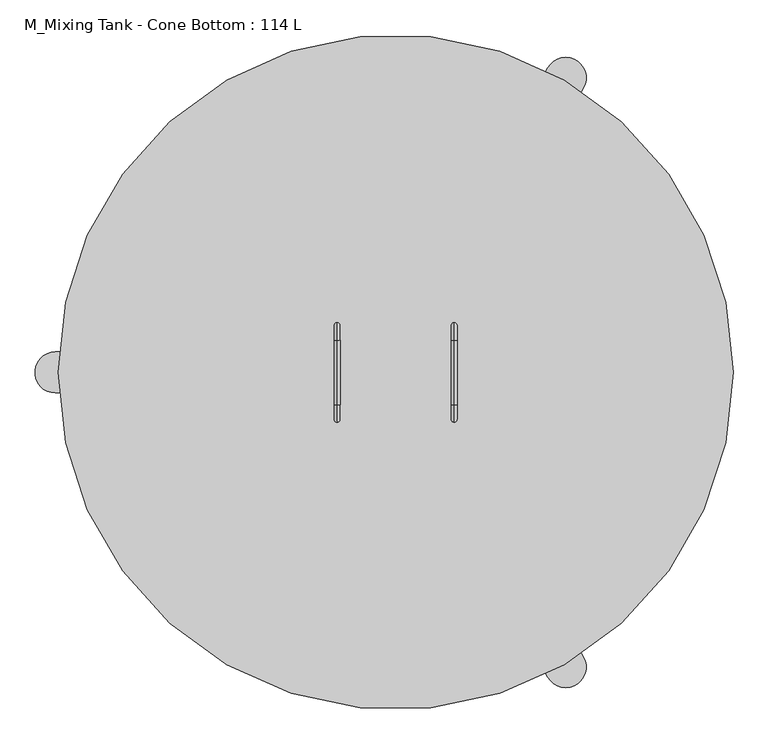
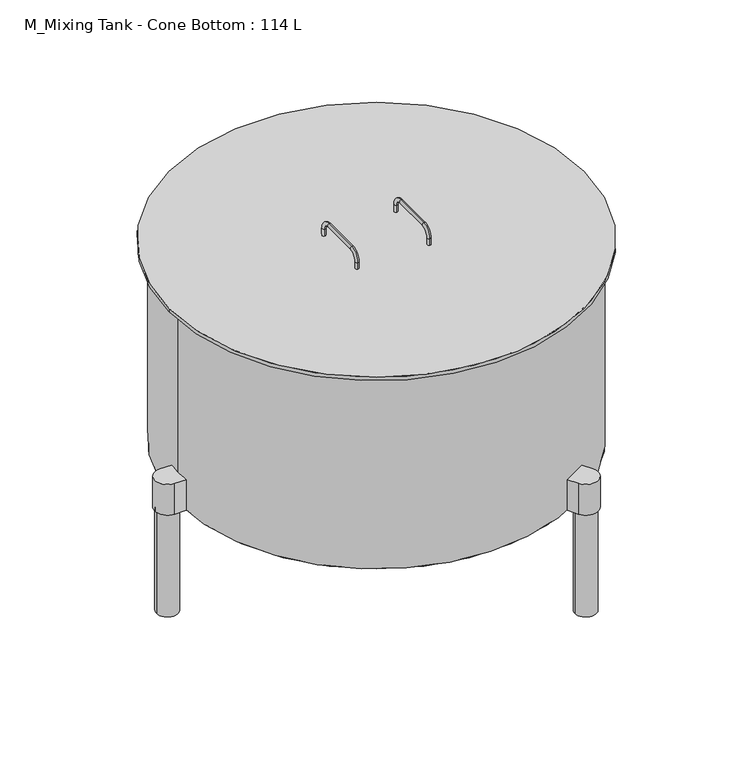
"""IFC4 building model written with IfcOpenShell, lengths in millimetres: proxy geometry, M_Mixing Tank - Cone Bottom : 114 L."""

import ifcopenshell
import ifcopenshell.guid

model = None  # the IFC model being written
_history = None  # IfcOwnerHistory: only IFC2X3 demands one
_inside = {}  # id of a spatial element -> (the spatial element, [elements in it])
_under = {}  # id of a project, library or spatial element -> (it, [spatial elements below it])
_declared = {}  # id of a project -> (the project, [libraries it declares])
_typed = {}  # id of a type object -> (the type object, [elements of that type])
_made_of = {}  # id of a material, layer set ... -> (it, [elements and type objects made of it])


def new_model(schema):
    """Start an empty IFC model of exactly this schema.

    Asked for "IFC4X3", IfcOpenShell would pick the latest addendum, in which some entities
    have other attributes; the version numbers below select the first issue.
    IFC2X3 requires an IfcOwnerHistory on every rooted entity: one is made here for all.
    """
    global model, _history
    if schema == "IFC4X3":
        model = ifcopenshell.file(schema_version=(4, 3, 0, 0))
    else:
        model = ifcopenshell.file(schema=schema)
    _inside.clear()
    _under.clear()
    _declared.clear()
    _typed.clear()
    _made_of.clear()
    _history = None
    if model.schema == "IFC2X3":
        org = make("IfcOrganization", Name="unknown")
        user = make(
            "IfcPersonAndOrganization",
            ThePerson=make("IfcPerson", FamilyName="unknown"),
            TheOrganization=org,
        )
        app = make(
            "IfcApplication",
            ApplicationDeveloper=org,
            Version="unknown",
            ApplicationFullName="unknown",
            ApplicationIdentifier="unknown",
        )
        _history = make(
            "IfcOwnerHistory",
            OwningUser=user,
            OwningApplication=app,
            ChangeAction="ADDED",
            CreationDate=0,
        )
    return model


def make(cls, **values):
    """One entity of the class cls with the attributes given. An attribute that is None is left unset."""
    return model.create_entity(
        cls, **{name: value for name, value in values.items() if value is not None}
    )


def rooted(cls, **values):
    """An entity with a GlobalId (a new one), such as an element, a storey or a relation."""
    return make(cls, GlobalId=ifcopenshell.guid.new(), OwnerHistory=_history, **values)


def si_unit(unit_type, name, prefix=None):
    """IfcSIUnit, for example si_unit("LENGTHUNIT", "METRE", prefix="MILLI")."""
    return make("IfcSIUnit", UnitType=unit_type, Prefix=prefix, Name=name)


def assignment(units):
    """IfcUnitAssignment: the units of a project."""
    return None if units is None else make("IfcUnitAssignment", Units=units)


def point(xyz):
    """IfcCartesianPoint."""
    return None if xyz is None else make("IfcCartesianPoint", Coordinates=xyz)


def direction(xyz):
    """IfcDirection."""
    return None if xyz is None else make("IfcDirection", DirectionRatios=xyz)


def frame(location, z_axis=None, x_axis=None):
    """IfcAxis2Placement3D, a coordinate frame: its origin and axes. An axis left out is left unset."""
    return make(
        "IfcAxis2Placement3D",
        Location=point(location),
        Axis=direction(z_axis),
        RefDirection=direction(x_axis),
    )


def frame_2d(location, x_axis=None):
    """IfcAxis2Placement2D, a coordinate frame in the plane: its origin and x axis."""
    return make(
        "IfcAxis2Placement2D", Location=point(location), RefDirection=direction(x_axis)
    )


def origin():
    """The frame at (0, 0, 0) with its axes left unset."""
    return frame((0.0, 0.0, 0.0))


def origin_with_axes():
    """The frame at (0, 0, 0) with the z axis (0, 0, 1) and the x axis (1, 0, 0) written out."""
    return frame((0.0, 0.0, 0.0), z_axis=(0.0, 0.0, 1.0), x_axis=(1.0, 0.0, 0.0))


def origin_2d():
    """The frame at (0, 0) in the plane with its x axis left unset."""
    return frame_2d((0.0, 0.0))


def place(relative_to, where):
    """IfcLocalPlacement: puts the frame where relative to a parent placement (None: the world)."""
    return make(
        "IfcLocalPlacement", PlacementRelTo=relative_to, RelativePlacement=where
    )


def context(
    kind, dimensions, precision=None, world=None, true_north=None, identifier=None
):
    """IfcGeometricRepresentationContext, for example the 3D "Model" context."""
    return make(
        "IfcGeometricRepresentationContext",
        ContextIdentifier=identifier,
        ContextType=kind,
        CoordinateSpaceDimension=dimensions,
        Precision=precision,
        WorldCoordinateSystem=world,
        TrueNorth=true_north,
    )


def project(units=None, contexts=None):
    """IfcProject with its units and contexts."""
    return rooted(
        "IfcProject",
        Name="project",
        RepresentationContexts=contexts,
        UnitsInContext=assignment(units),
    )


def spatial(cls, under=None, at=None, **own):
    """A site, building, storey or space (cls), placed at a placement, below another one or the project."""
    s = rooted(cls, ObjectPlacement=at, **own)
    if under is not None:
        _under.setdefault(under.id(), (under, []))[1].append(s)
    return s


def polyline(points):
    """IfcPolyline through the points."""
    return make("IfcPolyline", Points=[point(p) for p in points])


def circle_curve(where, radius):
    """IfcCircle in the frame where."""
    return make("IfcCircle", Position=where, Radius=radius)


def ellipse_curve(where, semi_axis1, semi_axis2):
    """IfcEllipse in the frame where."""
    return make(
        "IfcEllipse", Position=where, SemiAxis1=semi_axis1, SemiAxis2=semi_axis2
    )


def trimmed(basis, trim1, trim2, sense, master):
    """IfcTrimmedCurve: the piece of a basis curve between two trims."""
    return make(
        "IfcTrimmedCurve",
        BasisCurve=basis,
        Trim1=trim1,
        Trim2=trim2,
        SenseAgreement=sense,
        MasterRepresentation=master,
    )


def segment(curve, same_sense, transition):
    """IfcCompositeCurveSegment."""
    return make(
        "IfcCompositeCurveSegment",
        Transition=transition,
        SameSense=same_sense,
        ParentCurve=curve,
    )


def composite_curve(segments, self_intersect=None):
    """IfcCompositeCurve: segments joined end to end."""
    return make("IfcCompositeCurve", Segments=segments, SelfIntersect=self_intersect)


def outline(outer, holes=None, kind="AREA"):
    """IfcArbitraryClosedProfileDef: a profile drawn as a closed curve; with holes, ...WithVoids."""
    if holes is None:
        return make("IfcArbitraryClosedProfileDef", ProfileType=kind, OuterCurve=outer)
    return make(
        "IfcArbitraryProfileDefWithVoids",
        ProfileType=kind,
        OuterCurve=outer,
        InnerCurves=holes,
    )


def extrude(swept, where, along, depth):
    """IfcExtrudedAreaSolid: the profile swept, set in the frame where, extruded along a direction by depth."""
    return make(
        "IfcExtrudedAreaSolid",
        SweptArea=swept,
        Position=where,
        ExtrudedDirection=direction(along),
        Depth=depth,
    )


def shape(context_of_items, identifier, shape_type, items):
    """IfcShapeRepresentation: the items that make up one representation, for example the "Body"."""
    return make(
        "IfcShapeRepresentation",
        ContextOfItems=context_of_items,
        RepresentationIdentifier=identifier,
        RepresentationType=shape_type,
        Items=items,
    )


def source(mapping_origin, context_of_items, identifier, shape_type, items):
    """IfcRepresentationMap: a shape defined once, which mapped items show again and again."""
    return make(
        "IfcRepresentationMap",
        MappingOrigin=mapping_origin,
        MappedRepresentation=shape(context_of_items, identifier, shape_type, items),
    )


def transform(
    local_origin,
    x_axis=None,
    y_axis=None,
    z_axis=None,
    scale=None,
    scale2=None,
    scale3=None,
    uniform=True,
):
    """IfcCartesianTransformationOperator3D, or its non-uniform kind. x_axis, y_axis, z_axis: its Axis1, 2, 3."""
    if uniform:
        return make(
            "IfcCartesianTransformationOperator3D",
            Axis1=direction(x_axis),
            Axis2=direction(y_axis),
            LocalOrigin=point(local_origin),
            Scale=scale,
            Axis3=direction(z_axis),
        )
    return make(
        "IfcCartesianTransformationOperator3DnonUniform",
        Axis1=direction(x_axis),
        Axis2=direction(y_axis),
        LocalOrigin=point(local_origin),
        Scale=scale,
        Axis3=direction(z_axis),
        Scale2=scale2,
        Scale3=scale3,
    )


def mapped(mapping_source, mapping_target):
    """IfcMappedItem: shows the shape of a source again, moved by a transform."""
    return make(
        "IfcMappedItem", MappingSource=mapping_source, MappingTarget=mapping_target
    )


def made_of(thing, what):
    """Note that an element or type object is made of a material, layer set ...; save() writes the relation."""
    if what is not None:
        _made_of.setdefault(what.id(), (what, []))[1].append(thing)
    return thing


def element(
    cls,
    number,
    at=None,
    inside=None,
    cuts=None,
    type_object=None,
    material=None,
    context=None,
    identifier="Body",
    shape_type=None,
    held_by="IfcProductDefinitionShape",
    body=None,
    shapes=None,
    **own,
):
    """One element of the class cls, such as IfcWall. Its Tag is "e" and its number.

    at: its placement. inside: the storey or other place that contains it. cuts: it is an
    opening in that element (IfcRelVoidsElement). A single representation is given by context,
    identifier, shape_type and body (its items); several are given by shapes. held_by: the class
    of the entity that holds the representations. save() writes the other relations.
    """
    e = rooted(cls, Tag="e%d" % number, ObjectPlacement=at, **own)
    if body is not None:
        shapes = [shape(context, identifier, shape_type, body)]
    if shapes is not None:
        e.Representation = make(held_by, Representations=shapes)
    if inside is not None:
        _inside.setdefault(inside.id(), (inside, []))[1].append(e)
    if cuts is not None:
        rooted(
            "IfcRelVoidsElement", RelatingBuildingElement=cuts, RelatedOpeningElement=e
        )
    if type_object is not None:
        _typed.setdefault(type_object.id(), (type_object, []))[1].append(e)
    return made_of(e, material)


def aggregate(whole, parts):
    """IfcRelAggregates: a whole, such as a stair, and the parts it consists of."""
    return rooted("IfcRelAggregates", RelatingObject=whole, RelatedObjects=parts)


def save(model, path):
    """Write the relations noted so far, then the file.

    IfcRelAggregates (storeys below a building ...), IfcRelContainedInSpatialStructure (elements
    in a storey), IfcRelDefinesByType, IfcRelAssociatesMaterial and IfcRelDeclares: one each for
    every whole, place, type object, material and project.
    """
    for whole, parts in _under.values():
        aggregate(whole, parts)
    for where, things in _inside.values():
        rooted(
            "IfcRelContainedInSpatialStructure",
            RelatedElements=things,
            RelatingStructure=where,
        )
    for kind, things in _typed.values():
        rooted("IfcRelDefinesByType", RelatedObjects=things, RelatingType=kind)
    for what, things in _made_of.values():
        rooted("IfcRelAssociatesMaterial", RelatedObjects=things, RelatingMaterial=what)
    for by, libraries in _declared.values():
        rooted("IfcRelDeclares", RelatingContext=by, RelatedDefinitions=libraries)
    model.write(path)


def plane_surface(at):
    """IfcPlane: the flat surface through the origin of the frame at, square to its z axis."""
    return make("IfcPlane", Position=at)


def cylinder_surface(at, radius):
    """IfcCylindricalSurface: all points at the distance radius from the z axis of the frame at."""
    return make("IfcCylindricalSurface", Position=at, Radius=radius)


def revolved_surface(curve, axis_point, axis_direction):
    """IfcSurfaceOfRevolution: the curve turned about the line through axis_point along axis_direction."""
    return make(
        "IfcSurfaceOfRevolution",
        SweptCurve=make("IfcArbitraryOpenProfileDef", ProfileType="CURVE", Curve=curve),
        AxisPosition=make("IfcAxis1Placement", Location=point(axis_point), Axis=direction(axis_direction)),
    )


def advanced_brep(points, edges, surfaces, faces):
    """IfcAdvancedBrep: a solid bounded by faces that lie on surfaces and meet in shared edges.

    An edge is (start, end): straight between two places in points (the first is 0);
    or (start, end, curve); or (start, end, curve, False) where it runs against its curve.
    A face is (place in surfaces, loops), or (place, loops, False) where it looks against
    its surface's normal. A loop lists edges by number (the first is 1), with a minus sign
    where the edge is run from its end to its start. The first loop is the outer one.
    """
    corners = [point(p) for p in points]
    vertices = [make("IfcVertexPoint", VertexGeometry=c) for c in corners]
    made = []
    for start, end, *more in edges:
        made.append(
            make(
                "IfcEdgeCurve",
                EdgeStart=vertices[start],
                EdgeEnd=vertices[end],
                EdgeGeometry=more[0] if more else make("IfcPolyline", Points=[corners[start], corners[end]]),
                SameSense=more[1] if len(more) > 1 else True,
            )
        )
    hull = []
    for where, loops, *sense in faces:
        bounds = []
        for j, loop in enumerate(loops):
            ring = [make("IfcOrientedEdge", EdgeElement=made[abs(k) - 1], Orientation=k > 0) for k in loop]
            bounds.append(
                make(
                    "IfcFaceOuterBound" if j == 0 else "IfcFaceBound",
                    Bound=make("IfcEdgeLoop", EdgeList=ring),
                    Orientation=True,
                )
            )
        hull.append(make("IfcAdvancedFace", Bounds=bounds, FaceSurface=surfaces[where], SameSense=sense[0] if sense else True))
    return make("IfcAdvancedBrep", Outer=make("IfcClosedShell", CfsFaces=hull))


def m_mixing_tank_cone_bottom_114_l_11de7092(model_context):
    return source(origin(), model_context, "Body", "SolidModel", [
        extrude(outline(composite_curve([segment(trimmed(circle_curve(origin_2d(), 732.0), [point((-732.0, 0.0))], [point((732.0, 0.0))], False, "CARTESIAN"), True, "CONTINUOUS"), segment(trimmed(circle_curve(origin_2d(), 732.0), [point((732.0, 0.0))], [point((-732.0, 0.0))], False, "CARTESIAN"), True, "CONTINUOUS")], self_intersect=False)), frame((0.0, 0.0, 1108.3), z_axis=(0.0, 0.0, 1.0), x_axis=(1.0, 0.0, 0.0)), (0.0, 0.0, 1.0), 12.7),
        advanced_brep(
        [(700.0, 0.0, 384.0), (-700.0, 0.0, 384.0), (25.0, 0.0, 196.4355653), (-25.0, 0.0, 196.4355653)],
        [
            (0, 1, circle_curve(frame((0.0, 0.0, 384.0), z_axis=(0.0, 0.0, 1.0), x_axis=(1.0, 0.0, 0.0)), 700.0)),
            (1, 0, circle_curve(frame((0.0, 0.0, 384.0), z_axis=(0.0, 0.0, 1.0), x_axis=(-1.0, 0.0, 0.0)), 700.0)),
            (2, 3, circle_curve(frame((0.0, 0.0, 196.4355653), z_axis=(0.0, 0.0, -1.0), x_axis=(-1.0, 0.0, 0.0)), 25.0)),
            (3, 2, circle_curve(frame((0.0, 0.0, 196.4355653), z_axis=(0.0, 0.0, -1.0), x_axis=(1.0, 0.0, 0.0)), 25.0)),
            (3, 1),
            (0, 2),
        ],
        [
            plane_surface(frame((0.0, 0.0, 384.0), z_axis=(0.0, 0.0, 1.0), x_axis=(0.0, 1.0, 0.0))),
            plane_surface(frame((0.0, 0.0, 196.4355653), z_axis=(0.0, 0.0, -1.0), x_axis=(0.0, 1.0, 0.0))),
            revolved_surface(polyline([(-24.99999994858913, 0.0, 196.4355653), (-700.0, 0.0, 384.0)]), (0.0, 0.0, 189.4887344), (0.0, 0.0, 1.0)),
            revolved_surface(polyline([(24.99999994858913, 0.0, 196.4355653), (700.0, 0.0, 384.0)]), (0.0, 0.0, 189.4887344), (0.0, 0.0, 1.0)),
        ],
        [
            (0, [[1, 2]]),
            (1, [[3, 4]]),
            (2, [[-4, 5, -1, 6]]),
            (3, [[-3, -6, -2, -5]]),
        ],
    ),
        extrude(outline(composite_curve([segment(trimmed(circle_curve(origin_2d(), 25.0), [point((-25.0, 0.0))], [point((25.0, 0.0))], False, "CARTESIAN"), True, "CONTINUOUS"), segment(trimmed(circle_curve(origin_2d(), 25.0), [point((25.0, 0.0))], [point((-25.0, 0.0))], False, "CARTESIAN"), True, "CONTINUOUS")], self_intersect=False)), frame((0.0, 0.0, 167.0668153), z_axis=(0.0, 0.0, 1.0), x_axis=(1.0, 0.0, 0.0)), (0.0, 0.0, 1.0), 29.36875),
        extrude(outline(composite_curve([segment(trimmed(circle_curve(origin_2d(), 700.0), [point((-700.0, 0.0))], [point((700.0, 0.0))], False, "CARTESIAN"), True, "CONTINUOUS"), segment(trimmed(circle_curve(origin_2d(), 700.0), [point((700.0, 0.0))], [point((-700.0, 0.0))], False, "CARTESIAN"), True, "CONTINUOUS")], self_intersect=False)), frame((0.0, 0.0, 384.0), z_axis=(0.0, 0.0, 1.0), x_axis=(1.0, 0.0, 0.0)), (0.0, 0.0, 1.0), 724.3),
        extrude(outline(composite_curve([segment(polyline([(407.4948292, 616.901748), (387.1653983, 581.6901407)]), True, "CONTINUOUS"), segment(trimmed(circle_curve(origin_2d(), 698.7563706), [point((387.1653983, 581.6901407))], [point((310.1757399, 626.1401407))], True, "CARTESIAN"), True, "CONTINUOUS"), segment(polyline([(310.1757399, 626.1401407), (330.5051708, 661.351748)]), True, "CONTINUOUS"), segment(trimmed(circle_curve(frame_2d((369.0, 639.126748)), 44.45), [point((330.5051708, 661.351748))], [point((407.4948292, 616.901748))], False, "CARTESIAN"), True, "CONTINUOUS")], self_intersect=False)), frame((0.0, 0.0, 384.0), z_axis=(0.0, 0.0, 1.0), x_axis=(1.0, 0.0, 0.0)), (0.0, 0.0, 1.0), 114.475),
        extrude(outline(composite_curve([segment(trimmed(circle_curve(frame_2d((-738.0, 0.0)), 44.45), [point((-738.0, -44.45))], [point((-738.0, 44.45))], False, "CARTESIAN"), True, "CONTINUOUS"), segment(polyline([(-738.0, 44.45), (-697.3411382, 44.45)]), True, "CONTINUOUS"), segment(trimmed(circle_curve(origin_2d(), 698.7563706), [point((-697.3411382, 44.45))], [point((-697.3411382, -44.45))], True, "CARTESIAN"), True, "CONTINUOUS"), segment(polyline([(-697.3411382, -44.45), (-738.0, -44.45)]), True, "CONTINUOUS")], self_intersect=False)), frame((0.0, 0.0, 384.0), z_axis=(0.0, 0.0, 1.0), x_axis=(1.0, 0.0, 0.0)), (0.0, 0.0, 1.0), 114.475),
        extrude(outline(composite_curve([segment(trimmed(circle_curve(frame_2d((369.0, -639.126748)), 44.45), [point((407.4948292, -616.901748))], [point((330.5051708, -661.351748))], False, "CARTESIAN"), True, "CONTINUOUS"), segment(polyline([(330.5051708, -661.351748), (310.7988143, -627.2193373)]), True, "CONTINUOUS"), segment(trimmed(circle_curve(origin_2d(), 700.0), [point((310.7988143, -627.2193373))], [point((387.7884727, -582.7693373))], True, "CARTESIAN"), True, "CONTINUOUS"), segment(polyline([(387.7884727, -582.7693373), (407.4948292, -616.901748)]), True, "CONTINUOUS")], self_intersect=False)), frame((0.0, 0.0, 384.0), z_axis=(0.0, 0.0, 1.0), x_axis=(1.0, 0.0, 0.0)), (0.0, 0.0, 1.0), 114.475),
        extrude(outline(composite_curve([segment(trimmed(circle_curve(frame_2d((-738.0, 0.0)), 38.1), [point((-699.9, 0.0))], [point((-776.1, 0.0))], False, "CARTESIAN"), True, "CONTINUOUS"), segment(trimmed(circle_curve(frame_2d((-738.0, 0.0)), 38.1), [point((-776.1, 0.0))], [point((-699.9, 0.0))], False, "CARTESIAN"), True, "CONTINUOUS")], self_intersect=False)), origin_with_axes(), (0.0, 0.0, 1.0), 384.0),
        extrude(outline(composite_curve([segment(trimmed(circle_curve(frame_2d((369.0, 639.126748)), 38.1), [point((407.1, 639.126748))], [point((330.9, 639.126748))], False, "CARTESIAN"), True, "CONTINUOUS"), segment(trimmed(circle_curve(frame_2d((369.0, 639.126748)), 38.1), [point((330.9, 639.126748))], [point((407.1, 639.126748))], False, "CARTESIAN"), True, "CONTINUOUS")], self_intersect=False)), origin_with_axes(), (0.0, 0.0, 1.0), 384.0),
        extrude(outline(composite_curve([segment(trimmed(circle_curve(frame_2d((369.0, -639.126748)), 38.1), [point((407.1, -639.126748))], [point((330.9, -639.126748))], False, "CARTESIAN"), True, "CONTINUOUS"), segment(trimmed(circle_curve(frame_2d((369.0, -639.126748)), 38.1), [point((330.9, -639.126748))], [point((407.1, -639.126748))], False, "CARTESIAN"), True, "CONTINUOUS")], self_intersect=False)), origin_with_axes(), (0.0, 0.0, 1.0), 384.0),
        advanced_brep(
        [(127.0, 107.85, 1121.0), (127.0, 95.15, 1121.0), (127.0, 107.85, 1146.4), (127.0, 95.15, 1146.4), (127.0, 69.75, 1184.5), (127.0, 69.75, 1171.8), (127.0, -69.75, 1184.5), (127.0, -69.75, 1171.8), (127.0, -107.85, 1146.4), (127.0, -95.15, 1146.4), (127.0, -107.85, 1121.0), (127.0, -95.15, 1121.0)],
        [
            (0, 1, circle_curve(frame((127.0, 101.5, 1121.0), z_axis=(0.0, 0.0, -1.0), x_axis=(0.0, -1.0, 0.0)), 6.35)),
            (1, 0, circle_curve(frame((127.0, 101.5, 1121.0), z_axis=(0.0, 0.0, -1.0), x_axis=(0.0, -1.0, 0.0)), 6.35)),
            (0, 2),
            (2, 3, circle_curve(frame((127.0, 101.5, 1146.4), z_axis=(0.0, 0.0, -1.0), x_axis=(0.0, -1.0, 0.0)), 6.35)),
            (3, 1),
            (3, 2, circle_curve(frame((127.0, 101.5, 1146.4), z_axis=(0.0, 0.0, -1.0), x_axis=(0.0, -1.0, 0.0)), 6.35)),
            (2, 4, circle_curve(frame((127.0, 69.75, 1146.4), z_axis=(1.0, 0.0, 0.0), x_axis=(0.0, 1.0, 0.0)), 38.1)),
            (4, 5, circle_curve(frame((127.0, 69.75, 1178.15), z_axis=(0.0, 1.0, 0.0), x_axis=(0.0, 0.0, -1.0)), 6.35)),
            (5, 3, circle_curve(frame((127.0, 69.75, 1146.4), z_axis=(-1.0, 0.0, 0.0), x_axis=(0.0, 1.0, 0.0)), 25.4)),
            (5, 4, circle_curve(frame((127.0, 69.75, 1178.15), z_axis=(0.0, 1.0, 0.0), x_axis=(0.0, 0.0, -1.0)), 6.35)),
            (4, 6),
            (6, 7, circle_curve(frame((127.0, -69.75, 1178.15), z_axis=(0.0, 1.0, 0.0), x_axis=(0.0, 0.0, -1.0)), 6.35)),
            (7, 5),
            (7, 6, circle_curve(frame((127.0, -69.75, 1178.15), z_axis=(0.0, 1.0, 0.0), x_axis=(0.0, 0.0, -1.0)), 6.35)),
            (6, 8, circle_curve(frame((127.0, -69.75, 1146.4), z_axis=(1.0, 0.0, 0.0), x_axis=(0.0, 0.0, 1.0)), 38.1)),
            (8, 9, circle_curve(frame((127.0, -101.5, 1146.4), z_axis=(0.0, 0.0, 1.0), x_axis=(0.0, 1.0, 0.0)), 6.35)),
            (9, 7, circle_curve(frame((127.0, -69.75, 1146.4), z_axis=(-1.0, 0.0, 0.0), x_axis=(0.0, 0.0, 1.0)), 25.4)),
            (9, 8, circle_curve(frame((127.0, -101.5, 1146.4), z_axis=(0.0, 0.0, 1.0), x_axis=(0.0, 1.0, 0.0)), 6.35)),
            (10, 11, circle_curve(frame((127.0, -101.5, 1121.0), z_axis=(0.0, 0.0, -1.0), x_axis=(0.0, 1.0, 0.0)), 6.35)),
            (11, 10, circle_curve(frame((127.0, -101.5, 1121.0), z_axis=(0.0, 0.0, -1.0), x_axis=(0.0, 1.0, 0.0)), 6.35)),
            (8, 10),
            (11, 9),
        ],
        [
            plane_surface(frame((127.0, 101.5, 1121.0), z_axis=(0.0, 0.0, -1.0), x_axis=(1.0, 0.0, 0.0))),
            cylinder_surface(frame((127.0, 101.5, 1121.0), z_axis=(0.0, 0.0, -1.0), x_axis=(0.0, -1.0, 0.0)), 6.35),
            revolved_surface(trimmed(ellipse_curve(frame((127.0, 101.5, 1146.4), z_axis=(0.0, 0.0, -1.0), x_axis=(0.0, -1.0, 0.0)), 6.35, 6.35), [point((127.0, 107.85, 1146.4))], [point((127.0, 95.15, 1146.4))], True, "CARTESIAN"), (127.0, 69.75, 1146.4), (1.0, 0.0, 0.0)),
            revolved_surface(trimmed(ellipse_curve(frame((127.0, 101.5, 1146.4), z_axis=(0.0, 0.0, -1.0), x_axis=(0.0, -1.0, 0.0)), 6.35, 6.35), [point((127.0, 95.15, 1146.4))], [point((127.0, 107.85, 1146.4))], True, "CARTESIAN"), (127.0, 69.75, 1146.4), (1.0, 0.0, 0.0)),
            cylinder_surface(frame((127.0, 69.75, 1178.15), z_axis=(0.0, 1.0, 0.0), x_axis=(0.0, 0.0, -1.0)), 6.35),
            revolved_surface(trimmed(ellipse_curve(frame((127.0, -69.75, 1178.15), z_axis=(0.0, 1.0, 0.0), x_axis=(0.0, 0.0, -1.0)), 6.35, 6.35), [point((127.0, -69.75, 1184.5))], [point((127.0, -69.75, 1171.8))], True, "CARTESIAN"), (127.0, -69.75, 1146.4), (1.0, 0.0, 0.0)),
            revolved_surface(trimmed(ellipse_curve(frame((127.0, -69.75, 1178.15), z_axis=(0.0, 1.0, 0.0), x_axis=(0.0, 0.0, -1.0)), 6.35, 6.35), [point((127.0, -69.75, 1171.8))], [point((127.0, -69.75, 1184.5))], True, "CARTESIAN"), (127.0, -69.75, 1146.4), (1.0, 0.0, 0.0)),
            plane_surface(frame((127.0, -101.5, 1121.0), z_axis=(0.0, 0.0, -1.0), x_axis=(1.0, 0.0, 0.0))),
            cylinder_surface(frame((127.0, -101.5, 1146.4), z_axis=(0.0, 0.0, 1.0), x_axis=(0.0, 1.0, 0.0)), 6.35),
        ],
        [
            (0, [[1, 2]]),
            (1, [[-1, 3, 4, 5]]),
            (1, [[-2, -5, 6, -3]]),
            (2, [[-4, 7, 8, 9]]),
            (3, [[-6, -9, 10, -7]]),
            (4, [[-8, 11, 12, 13]]),
            (4, [[-10, -13, 14, -11]]),
            (5, [[-12, 15, 16, 17]]),
            (6, [[-14, -17, 18, -15]]),
            (7, [[19, 20]]),
            (8, [[-16, 21, -20, 22]]),
            (8, [[-18, -22, -19, -21]]),
        ],
    ),
        advanced_brep(
        [(-127.0, 107.85, 1121.0), (-127.0, 95.15, 1121.0), (-127.0, 107.85, 1146.4), (-127.0, 95.15, 1146.4), (-127.0, 69.75, 1184.5), (-127.0, 69.75, 1171.8), (-127.0, -69.75, 1184.5), (-127.0, -69.75, 1171.8), (-127.0, -107.85, 1146.4), (-127.0, -95.15, 1146.4), (-127.0, -107.85, 1121.0), (-127.0, -95.15, 1121.0)],
        [
            (0, 1, circle_curve(frame((-127.0, 101.5, 1121.0), z_axis=(0.0, 0.0, -1.0), x_axis=(0.0, -1.0, 0.0)), 6.35)),
            (1, 0, circle_curve(frame((-127.0, 101.5, 1121.0), z_axis=(0.0, 0.0, -1.0), x_axis=(0.0, -1.0, 0.0)), 6.35)),
            (0, 2),
            (2, 3, circle_curve(frame((-127.0, 101.5, 1146.4), z_axis=(0.0, 0.0, -1.0), x_axis=(0.0, -1.0, 0.0)), 6.35)),
            (3, 1),
            (3, 2, circle_curve(frame((-127.0, 101.5, 1146.4), z_axis=(0.0, 0.0, -1.0), x_axis=(0.0, -1.0, 0.0)), 6.35)),
            (2, 4, circle_curve(frame((-127.0, 69.75, 1146.4), z_axis=(1.0, 0.0, 0.0), x_axis=(0.0, 1.0, 0.0)), 38.1)),
            (4, 5, circle_curve(frame((-127.0, 69.75, 1178.15), z_axis=(0.0, 1.0, 0.0), x_axis=(0.0, 0.0, -1.0)), 6.35)),
            (5, 3, circle_curve(frame((-127.0, 69.75, 1146.4), z_axis=(-1.0, 0.0, 0.0), x_axis=(0.0, 1.0, 0.0)), 25.4)),
            (5, 4, circle_curve(frame((-127.0, 69.75, 1178.15), z_axis=(0.0, 1.0, 0.0), x_axis=(0.0, 0.0, -1.0)), 6.35)),
            (4, 6),
            (6, 7, circle_curve(frame((-127.0, -69.75, 1178.15), z_axis=(0.0, 1.0, 0.0), x_axis=(0.0, 0.0, -1.0)), 6.35)),
            (7, 5),
            (7, 6, circle_curve(frame((-127.0, -69.75, 1178.15), z_axis=(0.0, 1.0, 0.0), x_axis=(0.0, 0.0, -1.0)), 6.35)),
            (6, 8, circle_curve(frame((-127.0, -69.75, 1146.4), z_axis=(1.0, 0.0, 0.0), x_axis=(0.0, 0.0, 1.0)), 38.1)),
            (8, 9, circle_curve(frame((-127.0, -101.5, 1146.4), z_axis=(0.0, 0.0, 1.0), x_axis=(0.0, 1.0, 0.0)), 6.35)),
            (9, 7, circle_curve(frame((-127.0, -69.75, 1146.4), z_axis=(-1.0, 0.0, 0.0), x_axis=(0.0, 0.0, 1.0)), 25.4)),
            (9, 8, circle_curve(frame((-127.0, -101.5, 1146.4), z_axis=(0.0, 0.0, 1.0), x_axis=(0.0, 1.0, 0.0)), 6.35)),
            (10, 11, circle_curve(frame((-127.0, -101.5, 1121.0), z_axis=(0.0, 0.0, -1.0), x_axis=(0.0, 1.0, 0.0)), 6.35)),
            (11, 10, circle_curve(frame((-127.0, -101.5, 1121.0), z_axis=(0.0, 0.0, -1.0), x_axis=(0.0, 1.0, 0.0)), 6.35)),
            (8, 10),
            (11, 9),
        ],
        [
            plane_surface(frame((-127.0, 101.5, 1121.0), z_axis=(0.0, 0.0, -1.0), x_axis=(1.0, 0.0, 0.0))),
            cylinder_surface(frame((-127.0, 101.5, 1121.0), z_axis=(0.0, 0.0, -1.0), x_axis=(0.0, -1.0, 0.0)), 6.35),
            revolved_surface(trimmed(ellipse_curve(frame((-127.0, 101.5, 1146.4), z_axis=(0.0, 0.0, -1.0), x_axis=(0.0, -1.0, 0.0)), 6.35, 6.35), [point((-127.0, 107.85, 1146.4))], [point((-127.0, 95.15, 1146.4))], True, "CARTESIAN"), (-127.0, 69.75, 1146.4), (1.0, 0.0, 0.0)),
            revolved_surface(trimmed(ellipse_curve(frame((-127.0, 101.5, 1146.4), z_axis=(0.0, 0.0, -1.0), x_axis=(0.0, -1.0, 0.0)), 6.35, 6.35), [point((-127.0, 95.15, 1146.4))], [point((-127.0, 107.85, 1146.4))], True, "CARTESIAN"), (-127.0, 69.75, 1146.4), (1.0, 0.0, 0.0)),
            cylinder_surface(frame((-127.0, 69.75, 1178.15), z_axis=(0.0, 1.0, 0.0), x_axis=(0.0, 0.0, -1.0)), 6.35),
            revolved_surface(trimmed(ellipse_curve(frame((-127.0, -69.75, 1178.15), z_axis=(0.0, 1.0, 0.0), x_axis=(0.0, 0.0, -1.0)), 6.35, 6.35), [point((-127.0, -69.75, 1184.5))], [point((-127.0, -69.75, 1171.8))], True, "CARTESIAN"), (-127.0, -69.75, 1146.4), (1.0, 0.0, 0.0)),
            revolved_surface(trimmed(ellipse_curve(frame((-127.0, -69.75, 1178.15), z_axis=(0.0, 1.0, 0.0), x_axis=(0.0, 0.0, -1.0)), 6.35, 6.35), [point((-127.0, -69.75, 1171.8))], [point((-127.0, -69.75, 1184.5))], True, "CARTESIAN"), (-127.0, -69.75, 1146.4), (1.0, 0.0, 0.0)),
            plane_surface(frame((-127.0, -101.5, 1121.0), z_axis=(0.0, 0.0, -1.0), x_axis=(1.0, 0.0, 0.0))),
            cylinder_surface(frame((-127.0, -101.5, 1146.4), z_axis=(0.0, 0.0, 1.0), x_axis=(0.0, 1.0, 0.0)), 6.35),
        ],
        [
            (0, [[1, 2]]),
            (1, [[-1, 3, 4, 5]]),
            (1, [[-2, -5, 6, -3]]),
            (2, [[-4, 7, 8, 9]]),
            (3, [[-6, -9, 10, -7]]),
            (4, [[-8, 11, 12, 13]]),
            (4, [[-10, -13, 14, -11]]),
            (5, [[-12, 15, 16, 17]]),
            (6, [[-14, -17, 18, -15]]),
            (7, [[19, 20]]),
            (8, [[-16, 21, -20, 22]]),
            (8, [[-18, -22, -19, -21]]),
        ],
    ),
    ])


if __name__ == "__main__":
    model = new_model("IFC4")
    model_context = context("Model", 3, world=origin())
    ifc_project = project(units=[si_unit("LENGTHUNIT", "METRE", prefix="MILLI")], contexts=[model_context])
    site = spatial("IfcSite", under=ifc_project)
    building = spatial("IfcBuilding", under=site)
    placement = place(None, origin())
    m_mixing_tank_cone_bottom_114_l_shape = m_mixing_tank_cone_bottom_114_l_11de7092(model_context)
    element("IfcBuildingElementProxy", 1, Name="M_Mixing Tank - Cone Bottom : 114 L", ObjectType="M_Mixing Tank - Cone Bottom : 114 L", at=placement, inside=building, context=model_context, shape_type="MappedRepresentation", body=[
        mapped(m_mixing_tank_cone_bottom_114_l_shape, transform((0.0, 0.0, 0.0), x_axis=(1.0, 0.0, 0.0), y_axis=(0.0, 1.0, 0.0), z_axis=(0.0, 0.0, 1.0))),
    ])
    save(model, "model.ifc")

# Revit data of these elements
# Type "M_Mixing Tank - Cone Bottom : 114 L"
#   Tank Radius = 0.7 m
#   Tank Height = 0.737 m
#   Pressure Drop [instance default] = 69000.0 Pa
#   Outlet Radius = 25 mm
#   Outlet Diameter = 50 mm
#   Leg Offset Vertical = 0.639127 m
#   Leg Offset Horizontal = 0.369 m
#   Leg Offset = 0.738 m
#   Leg Height = 0.384 m
#   Handrail Length = 0.203 m
#   Handrail Distance = 0.254 m
#   Flow [instance default] = 0.63 L/s
#   Cap Radius = 0.732 m
#   Bottom Offset = 0.187564 m
#   Tank material = none
#   Leg material = none
